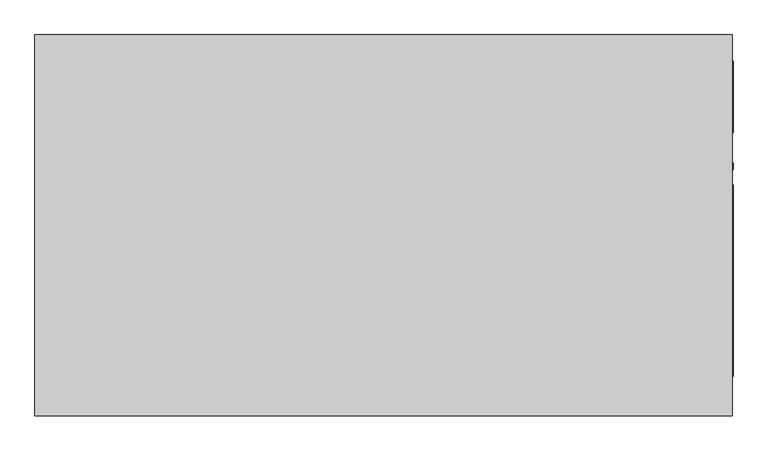
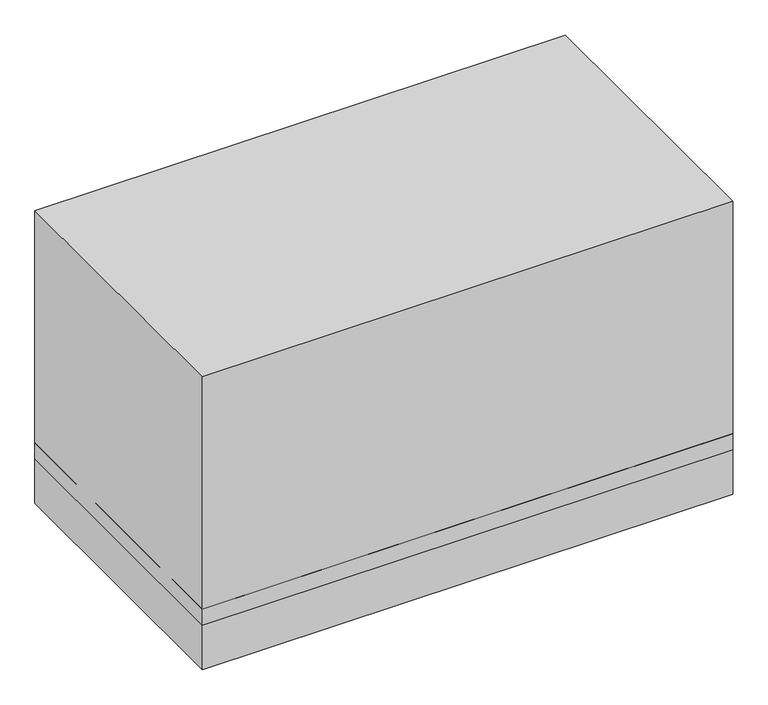
"""IFC4 building model written with IfcOpenShell, lengths in millimetres: proxy geometry, Carrier_48TC_Standard_Efficiency_Gas_Heat_Electric_Cooling_Packaged_Rooftop_Unit_3_to_15_nominal_tons : 15 ton 48TC**16."""

from ifc_helpers import new_model, si_unit, point, frame, frame_2d, origin, origin_with_axes, place, context, project, spatial, polyline, circle_curve, trimmed, segment, composite_curve, outline, extrude, source, transform, mapped, element, save
from ifc_brep_helpers import plane_surface, revolved_surface, advanced_brep


def mechanical_equipment_03f9c560(model_context):
    return source(origin(), model_context, "Body", "SolidModel", [
        extrude(outline(composite_curve([segment(trimmed(circle_curve(frame_2d((249.2375, 434.975)), 13.2953125), [point((235.9421875, 434.975))], [point((262.5328125, 434.975))], False, "CARTESIAN"), True, "CONTINUOUS"), segment(trimmed(circle_curve(frame_2d((249.2375, 434.975)), 13.2953125), [point((262.5328125, 434.975))], [point((235.9421875, 434.975))], False, "CARTESIAN"), True, "CONTINUOUS")], self_intersect=False)), frame((1471.6125, 0.0, 0.0), z_axis=(1.0, 0.0, 0.0), x_axis=(0.0, 1.0, 0.0)), (0.0, 0.0, 1.0), 3.175),
        advanced_brep(
        [(1471.6125, 804.8625, 1717.675), (-1471.6125, 804.8625, 1717.675), (-1471.6125, -804.8625, 1717.675), (1471.6125, -804.8625, 1717.675), (1471.6125, 804.8625, 260.35), (1471.6125, -804.8625, 260.35), (-1471.6125, -804.8625, 260.35), (-1471.6125, 804.8625, 260.35), (1312.8625, -681.0375, 260.35), (1312.8625, 182.5625, 260.35), (633.4125, 182.5625, 260.35), (633.4125, -681.0375, 260.35), (1312.8625, 642.9375, 260.35), (122.2375, 642.9375, 260.35), (122.2375, 322.2625, 260.35), (1312.8625, 322.2625, 260.35), (430.8078125, -144.4625, 260.35), (404.2171875, -144.4625, 260.35), (-336.55, -423.8625, 260.35), (-358.775, -423.8625, 260.35), (-315.9125, -344.4875, 260.35), (-379.4125, -344.4875, 260.35), (-325.4375, -233.3625, 260.35), (-369.8875, -233.3625, 260.35), (1312.8625, -681.0375, 381.0), (633.4125, -681.0375, 381.0), (633.4125, 182.5625, 381.0), (1312.8625, 182.5625, 381.0), (1312.8625, 642.9375, 381.0), (1312.8625, 322.2625, 381.0), (122.2375, 322.2625, 381.0), (122.2375, 642.9375, 381.0), (430.8078125, -144.4625, 415.925), (404.2171875, -144.4625, 415.925), (-336.55, -423.8625, 415.925), (-358.775, -423.8625, 415.925), (-315.9125, -344.4875, 415.925), (-379.4125, -344.4875, 415.925), (-325.4375, -233.3625, 415.925), (-369.8875, -233.3625, 415.925)],
        [
            (0, 1),
            (1, 2),
            (2, 3),
            (3, 0),
            (4, 5),
            (5, 6),
            (6, 7),
            (7, 4),
            (8, 9),
            (9, 10),
            (10, 11),
            (11, 8),
            (12, 13),
            (13, 14),
            (14, 15),
            (15, 12),
            (16, 17, circle_curve(frame((417.5125, -144.4625, 260.35), z_axis=(0.0, 0.0, 1.0), x_axis=(-1.0, 0.0, 0.0)), 13.2953125)),
            (17, 16, circle_curve(frame((417.5125, -144.4625, 260.35), z_axis=(0.0, 0.0, 1.0), x_axis=(-1.0, 0.0, 0.0)), 13.2953125)),
            (18, 19, circle_curve(frame((-347.6625, -423.8625, 260.35), z_axis=(0.0, 0.0, 1.0), x_axis=(-1.0, 0.0, 0.0)), 11.1125)),
            (19, 18, circle_curve(frame((-347.6625, -423.8625, 260.35), z_axis=(0.0, 0.0, 1.0), x_axis=(-1.0, 0.0, 0.0)), 11.1125)),
            (20, 21, circle_curve(frame((-347.6625, -344.4875, 260.35), z_axis=(0.0, 0.0, 1.0), x_axis=(-1.0, 0.0, 0.0)), 31.75)),
            (21, 20, circle_curve(frame((-347.6625, -344.4875, 260.35), z_axis=(0.0, 0.0, 1.0), x_axis=(-1.0, 0.0, 0.0)), 31.75)),
            (22, 23, circle_curve(frame((-347.6625, -233.3625, 260.35), z_axis=(0.0, 0.0, 1.0), x_axis=(-1.0, 0.0, 0.0)), 22.225)),
            (23, 22, circle_curve(frame((-347.6625, -233.3625, 260.35), z_axis=(0.0, 0.0, 1.0), x_axis=(-1.0, 0.0, 0.0)), 22.225)),
            (0, 4),
            (7, 1),
            (6, 2),
            (5, 3),
            (24, 25),
            (25, 26),
            (26, 27),
            (27, 24),
            (27, 9),
            (8, 24),
            (26, 10),
            (25, 11),
            (28, 29),
            (29, 30),
            (30, 31),
            (31, 28),
            (31, 13),
            (12, 28),
            (30, 14),
            (29, 15),
            (32, 33, circle_curve(frame((417.5125, -144.4625, 415.925), z_axis=(0.0, 0.0, -1.0), x_axis=(-1.0, 0.0, 0.0)), 13.2953125)),
            (33, 32, circle_curve(frame((417.5125, -144.4625, 415.925), z_axis=(0.0, 0.0, -1.0), x_axis=(-1.0, 0.0, 0.0)), 13.2953125)),
            (33, 17),
            (16, 32),
            (34, 35, circle_curve(frame((-347.6625, -423.8625, 415.925), z_axis=(0.0, 0.0, -1.0), x_axis=(-1.0, 0.0, 0.0)), 11.1125)),
            (35, 34, circle_curve(frame((-347.6625, -423.8625, 415.925), z_axis=(0.0, 0.0, -1.0), x_axis=(-1.0, 0.0, 0.0)), 11.1125)),
            (35, 19),
            (18, 34),
            (36, 37, circle_curve(frame((-347.6625, -344.4875, 415.925), z_axis=(0.0, 0.0, -1.0), x_axis=(-1.0, 0.0, 0.0)), 31.75)),
            (37, 36, circle_curve(frame((-347.6625, -344.4875, 415.925), z_axis=(0.0, 0.0, -1.0), x_axis=(-1.0, 0.0, 0.0)), 31.75)),
            (37, 21),
            (20, 36),
            (38, 39, circle_curve(frame((-347.6625, -233.3625, 415.925), z_axis=(0.0, 0.0, -1.0), x_axis=(-1.0, 0.0, 0.0)), 22.225)),
            (39, 38, circle_curve(frame((-347.6625, -233.3625, 415.925), z_axis=(0.0, 0.0, -1.0), x_axis=(-1.0, 0.0, 0.0)), 22.225)),
            (39, 23),
            (22, 38),
        ],
        [
            plane_surface(frame((-1471.6125, 804.8625, 1717.675), z_axis=(0.0, 0.0, 1.0), x_axis=(-1.0, 0.0, 0.0))),
            plane_surface(frame((-1471.6125, 804.8625, 260.35), z_axis=(0.0, 0.0, -1.0), x_axis=(1.0, 0.0, 0.0))),
            plane_surface(frame((1471.6125, 804.8625, 1717.675), z_axis=(0.0, 1.0, 0.0), x_axis=(0.0, 0.0, -1.0))),
            plane_surface(frame((-1471.6125, 804.8625, 1717.675), z_axis=(-1.0, 0.0, 0.0), x_axis=(0.0, 0.0, -1.0))),
            plane_surface(frame((-1471.6125, -804.8625, 1717.675), z_axis=(0.0, -1.0, 0.0), x_axis=(0.0, 0.0, -1.0))),
            plane_surface(frame((1471.6125, -804.8625, 1717.675), z_axis=(1.0, 0.0, 0.0), x_axis=(0.0, 0.0, -1.0))),
            plane_surface(frame((1312.8625, -681.0375, 381.0), z_axis=(0.0, 0.0, -1.0), x_axis=(0.0, 1.0, 0.0))),
            plane_surface(frame((1312.8625, -681.0375, 381.0), z_axis=(-1.0, 0.0, 0.0), x_axis=(0.0, 0.0, -1.0))),
            plane_surface(frame((1312.8625, 182.5625, 381.0), z_axis=(0.0, -1.0, 0.0), x_axis=(0.0, 0.0, -1.0))),
            plane_surface(frame((633.4125, 182.5625, 381.0), z_axis=(1.0, 0.0, 0.0), x_axis=(0.0, 0.0, -1.0))),
            plane_surface(frame((633.4125, -681.0375, 381.0), z_axis=(0.0, 1.0, 0.0), x_axis=(0.0, 0.0, -1.0))),
            plane_surface(frame((122.2375, 642.9375, 381.0), z_axis=(0.0, 0.0, -1.0), x_axis=(-1.0, 0.0, 0.0))),
            plane_surface(frame((1312.8625, 642.9375, 381.0), z_axis=(0.0, -1.0, 0.0), x_axis=(0.0, 0.0, -1.0))),
            plane_surface(frame((122.2375, 642.9375, 381.0), z_axis=(1.0, 0.0, 0.0), x_axis=(0.0, 0.0, -1.0))),
            plane_surface(frame((122.2375, 322.2625, 381.0), z_axis=(0.0, 1.0, 0.0), x_axis=(0.0, 0.0, -1.0))),
            plane_surface(frame((1312.8625, 322.2625, 381.0), z_axis=(-1.0, 0.0, 0.0), x_axis=(0.0, 0.0, -1.0))),
            plane_surface(frame((404.2171875, -144.4625, 415.925), z_axis=(0.0, 0.0, -1.0), x_axis=(0.0, -1.0, 0.0))),
            revolved_surface(polyline([(404.21718749999997, -144.4625, 415.925), (404.21718749999997, -144.4625, 260.35)]), (417.5125, -144.4625, 0.0), (0.0, 0.0, 1.0)),
            plane_surface(frame((-358.775, -423.8625, 415.925), z_axis=(0.0, 0.0, -1.0), x_axis=(0.0, -1.0, 0.0))),
            revolved_surface(polyline([(-358.77500000000003, -423.8625, 415.925), (-358.77500000000003, -423.8625, 260.35)]), (-347.6625, -423.8625, 0.0), (0.0, 0.0, 1.0)),
            plane_surface(frame((-379.4125, -344.4875, 415.925), z_axis=(0.0, 0.0, -1.0), x_axis=(0.0, -1.0, 0.0))),
            revolved_surface(polyline([(-379.4125, -344.4875, 415.925), (-379.4125, -344.4875, 260.35)]), (-347.6625, -344.4875, 0.0), (0.0, 0.0, 1.0)),
            plane_surface(frame((-369.8875, -233.3625, 415.925), z_axis=(0.0, 0.0, -1.0), x_axis=(0.0, -1.0, 0.0))),
            revolved_surface(polyline([(-369.88750000000005, -233.3625, 415.925), (-369.88750000000005, -233.3625, 260.35)]), (-347.6625, -233.3625, 0.0), (0.0, 0.0, 1.0)),
        ],
        [
            (0, [[1, 2, 3, 4]]),
            (1, [[5, 6, 7, 8], [9, 10, 11, 12], [13, 14, 15, 16], [17, 18], [19, 20], [21, 22], [23, 24]]),
            (2, [[-1, 25, -8, 26]]),
            (3, [[-2, -26, -7, 27]]),
            (4, [[-3, -27, -6, 28]]),
            (5, [[-4, -28, -5, -25]]),
            (6, [[29, 30, 31, 32]]),
            (7, [[-32, 33, -9, 34]]),
            (8, [[-31, 35, -10, -33]]),
            (9, [[-30, 36, -11, -35]]),
            (10, [[-29, -34, -12, -36]]),
            (11, [[37, 38, 39, 40]]),
            (12, [[-40, 41, -13, 42]]),
            (13, [[-39, 43, -14, -41]]),
            (14, [[-38, 44, -15, -43]]),
            (15, [[-37, -42, -16, -44]]),
            (16, [[45, 46]]),
            (17, [[-46, 47, -17, 48]]),
            (17, [[-45, -48, -18, -47]]),
            (18, [[49, 50]]),
            (19, [[-50, 51, -19, 52]]),
            (19, [[-49, -52, -20, -51]]),
            (20, [[53, 54]]),
            (21, [[-54, 55, -21, 56]]),
            (21, [[-53, -56, -22, -55]]),
            (22, [[57, 58]]),
            (23, [[-58, 59, -23, 60]]),
            (23, [[-57, -60, -24, -59]]),
        ],
    ),
        extrude(outline(polyline([(1471.6125, 804.8625), (1471.6125, -804.8625), (-1471.6125, -804.8625), (-1471.6125, 804.8625), (1471.6125, 804.8625)]), holes=[polyline([(1312.8625, 642.9375), (122.2375, 642.9375), (122.2375, 322.2625), (1312.8625, 322.2625), (1312.8625, 642.9375)]), polyline([(1312.8625, -681.0375), (1312.8625, 182.5625), (633.4125, 182.5625), (633.4125, -681.0375), (1312.8625, -681.0375)]), composite_curve([segment(trimmed(circle_curve(frame_2d((417.5125, -144.4625)), 13.2953125), [point((430.8078125, -144.4625))], [point((404.2171875, -144.4625))], True, "CARTESIAN"), True, "CONTINUOUS"), segment(trimmed(circle_curve(frame_2d((417.5125, -144.4625)), 13.2953125), [point((404.2171875, -144.4625))], [point((430.8078125, -144.4625))], True, "CARTESIAN"), True, "CONTINUOUS")], self_intersect=False), composite_curve([segment(trimmed(circle_curve(frame_2d((-347.6625, -423.8625)), 11.1125), [point((-336.55, -423.8625))], [point((-358.775, -423.8625))], True, "CARTESIAN"), True, "CONTINUOUS"), segment(trimmed(circle_curve(frame_2d((-347.6625, -423.8625)), 11.1125), [point((-358.775, -423.8625))], [point((-336.55, -423.8625))], True, "CARTESIAN"), True, "CONTINUOUS")], self_intersect=False), composite_curve([segment(trimmed(circle_curve(frame_2d((-347.6625, -344.4875)), 31.75), [point((-315.9125, -344.4875))], [point((-379.4125, -344.4875))], True, "CARTESIAN"), True, "CONTINUOUS"), segment(trimmed(circle_curve(frame_2d((-347.6625, -344.4875)), 31.75), [point((-379.4125, -344.4875))], [point((-315.9125, -344.4875))], True, "CARTESIAN"), True, "CONTINUOUS")], self_intersect=False), composite_curve([segment(trimmed(circle_curve(frame_2d((-347.6625, -233.3625)), 22.225), [point((-325.4375, -233.3625))], [point((-369.8875, -233.3625))], True, "CARTESIAN"), True, "CONTINUOUS"), segment(trimmed(circle_curve(frame_2d((-347.6625, -233.3625)), 22.225), [point((-369.8875, -233.3625))], [point((-325.4375, -233.3625))], True, "CARTESIAN"), True, "CONTINUOUS")], self_intersect=False)]), origin_with_axes(), (0.0, 0.0, 1.0), 355.6),
        extrude(outline(polyline([(1474.7875, 693.7375), (1474.7875, 392.1125), (1471.6125, 392.1125), (1471.6125, 693.7375), (1474.7875, 693.7375)])), frame((0.0, 0.0, 415.925), z_axis=(0.0, 0.0, 1.0), x_axis=(1.0, 0.0, 0.0)), (0.0, 0.0, 1.0), 1171.575),
        extrude(outline(polyline([(1474.7875, 169.8625), (1474.7875, -636.5875), (1471.6125, -636.5875), (1471.6125, 169.8625), (1474.7875, 169.8625)])), frame((0.0, 0.0, 415.925), z_axis=(0.0, 0.0, 1.0), x_axis=(1.0, 0.0, 0.0)), (0.0, 0.0, 1.0), 371.475),
    ])


if __name__ == "__main__":
    model = new_model("IFC4")
    model_context = context("Model", 3, world=origin())
    ifc_project = project(units=[si_unit("LENGTHUNIT", "METRE", prefix="MILLI")], contexts=[model_context])
    site = spatial("IfcSite", under=ifc_project)
    building = spatial("IfcBuilding", under=site)
    placement = place(None, origin())
    mechanical_equipment_shape = mechanical_equipment_03f9c560(model_context)
    element("IfcBuildingElementProxy", 1, Name="Carrier_48TC_Standard_Efficiency_Gas_Heat_Electric_Cooling_Packaged_Rooftop_Unit_3_to_15_nominal_tons : 15 ton 48TC**16", ObjectType="Carrier_48TC_Standard_Efficiency_Gas_Heat_Electric_Cooling_Packaged_Rooftop_Unit_3_to_15_nominal_tons : 15 ton 48TC**16", at=placement, inside=building, context=model_context, shape_type="MappedRepresentation", body=[
        mapped(mechanical_equipment_shape, transform((0.0, 0.0, 0.0), x_axis=(1.0, 0.0, 0.0), y_axis=(0.0, 1.0, 0.0), z_axis=(0.0, 0.0, 1.0))),
    ])
    save(model, "model.ifc")

# Revit data of these elements
# Type "Carrier_48TC_Standard_Efficiency_Gas_Heat_Electric_Cooling_Packaged_Rooftop_Unit_3_to_15_nominal_tons : 15 ton 48TC**16"
#   URL = "www.Carrier.com"
#   Model = "48TC"
#   Manufacturer = "Carrier"
#   Disclaimer = "Manufacturer reserves the right to change, at any time, specifications and designs without notice and without obligation.  Please verify critical parameters with local Carrier commercial sales office."
#   knockout thickness = 0' - 0 1/16"
#   Voltage = 0 V
#   Version = 1
#   TTBY3 = 1' - 3"
#   TTBY2 = 1' - 6 1/8"
#   TTBY1 = 1' - 10 1/2"
#   TTBX = 3' - 8 1/4"
#   TTBPowerR = 0' - 1 1/4"
#   TTBGasR = 0' - 0 7/8"
#   SSSZ = 0' - 6 1/8"
#   SSSY = 0' - 6 5/8"
#   SSSW = 2' - 7 3/4"
#   SSSH = 1' - 2 5/8"
#   SSRZ = 0' - 6 1/8"
#   SSRY = 0' - 4 3/8"
#   SSRW = 0' - 11 7/8"
#   SSRH = 3' - 10 1/8"
#   SEER = 0
#   Right clearance = 3' - 0"
#   PWRZ = 2' - 11 3/4"
#   PWRY = 0' - 11.71105"
#   PWRR = 0' - 1 1/4"
#   ODF2X = 2' - 1"
#   ODF1Y = 1' - 0"
#   ODF1X = 1' - 1"
#   ODF1R = 0' - 11"
#   MOCP = 0 A
#   MCA = 0 A
#   Left clearance = 4' - 0"
#   IEER = 11.7
#   Front clearance = 4' - 0"
#   Fan Z = 5' - 7 5/8"
#   Width = 5' - 3 3/8"
#   Length = 9' - 7 7/8"
#   Height = 4' - 9 3/8"
#   EER = 10.8
#   DSSY = 0' - 4 7/8"
#   DSSX = 0' - 6 1/4"
#   DSSW = 2' - 2 3/4"
#   DSSH = 2' - 10"
#   DSRY = 0' - 6 3/8"
#   DSRX = 0' - 6 1/4"
#   DSRW = 3' - 10 7/8"
#   DSRH = 1' - 0 5/8"
#   DRNZ = 0' - 6 7/8"
#   DRNY = 3' - 5 1/2"
#   DRNR = 0' - 0 67/128"
#   Curb Z = 1' - 2"
#   CFM (nominal) = 0 CFM
#   Back clearance = 3' - 0"
#   Alt Condensate Drain = 0' - 0 67/128"
#   AccypwrR = 0' - 0 7/16"
#   ACY = 2' - 2"
#   ACX = 3' - 5 1/2"
#   Gas [instance default] = yes
#   Fan 2 on = yes
#   Curb_1SLAB_2ROOFCURB_3SNOWCURB = 2
#   Fan 3 on = yes
#   Unit material = RTU
#   Curb material = Curb paint
# Element 1 (IfcBuildingElementProxy, "Carrier_48TC_Standard_Efficiency_Gas_Heat_Electric_Cooling_Packaged_Rooftop_Unit_3_to_15_nominal_tons : 15 ton 48TC**16")
#   Materials on its faces: "RTU", "Curb paint", "Mech"
# Materials
#   "RTU": class "Miscellaneous", colour RGB 104 104 104, transparency 0, Cost = 0
#   "Curb paint": class "Miscellaneous", colour RGB 189 187 185, transparency 0
#   "Mech": class "Miscellaneous", colour RGB 235 237 235, transparency 0, Cost = 0
